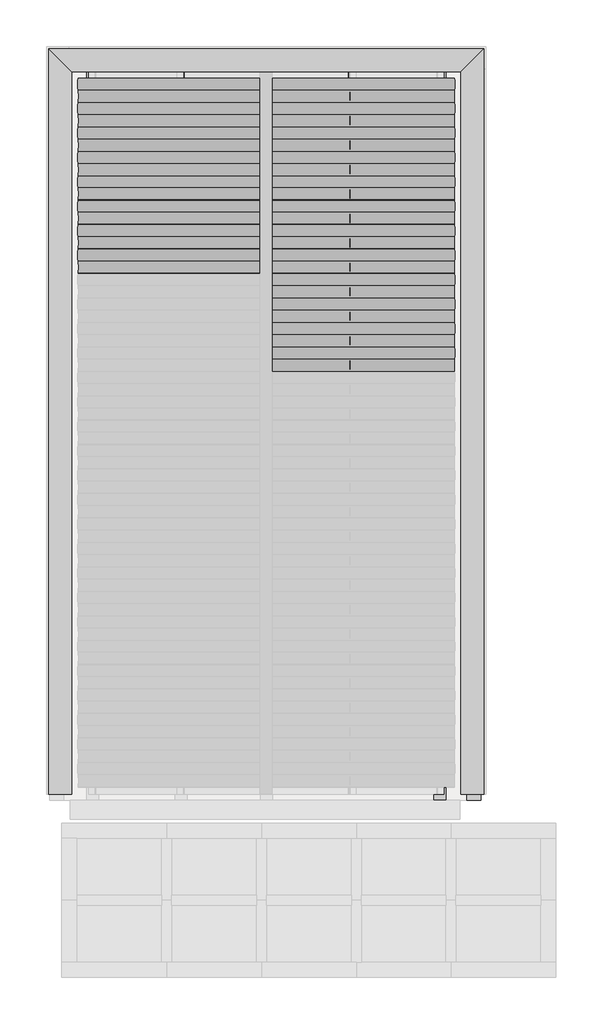
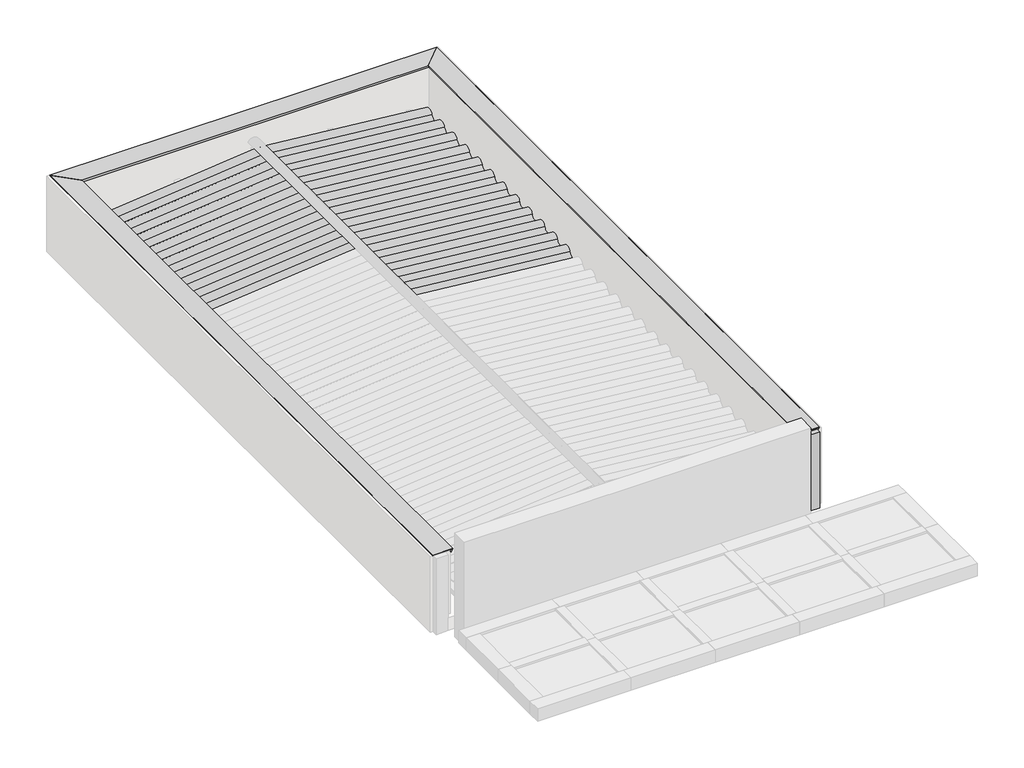
# One storey, part 3 of 3: 35 beams, 12 columns, 1 proxy.
"""IFC4 building model written with IfcOpenShell, lengths in millimetres."""

import ifcopenshell
import ifcopenshell.guid

model = None  # the IFC model being written
_history = None  # IfcOwnerHistory: only IFC2X3 demands one
_inside = {}  # id of a spatial element -> (the spatial element, [elements in it])
_under = {}  # id of a project, library or spatial element -> (it, [spatial elements below it])
_declared = {}  # id of a project -> (the project, [libraries it declares])
_typed = {}  # id of a type object -> (the type object, [elements of that type])
_made_of = {}  # id of a material, layer set ... -> (it, [elements and type objects made of it])


def new_model(schema):
    """Start an empty IFC model of exactly this schema.

    Asked for "IFC4X3", IfcOpenShell would pick the latest addendum, in which some entities
    have other attributes; the version numbers below select the first issue.
    IFC2X3 requires an IfcOwnerHistory on every rooted entity: one is made here for all.
    """
    global model, _history
    if schema == "IFC4X3":
        model = ifcopenshell.file(schema_version=(4, 3, 0, 0))
    else:
        model = ifcopenshell.file(schema=schema)
    _inside.clear()
    _under.clear()
    _declared.clear()
    _typed.clear()
    _made_of.clear()
    _history = None
    if model.schema == "IFC2X3":
        org = make("IfcOrganization", Name="unknown")
        user = make(
            "IfcPersonAndOrganization",
            ThePerson=make("IfcPerson", FamilyName="unknown"),
            TheOrganization=org,
        )
        app = make(
            "IfcApplication",
            ApplicationDeveloper=org,
            Version="unknown",
            ApplicationFullName="unknown",
            ApplicationIdentifier="unknown",
        )
        _history = make(
            "IfcOwnerHistory",
            OwningUser=user,
            OwningApplication=app,
            ChangeAction="ADDED",
            CreationDate=0,
        )
    return model


def make(cls, **values):
    """One entity of the class cls with the attributes given. An attribute that is None is left unset."""
    return model.create_entity(
        cls, **{name: value for name, value in values.items() if value is not None}
    )


def rooted(cls, **values):
    """An entity with a GlobalId (a new one), such as an element, a storey or a relation."""
    return make(cls, GlobalId=ifcopenshell.guid.new(), OwnerHistory=_history, **values)


def si_unit(unit_type, name, prefix=None):
    """IfcSIUnit, for example si_unit("LENGTHUNIT", "METRE", prefix="MILLI")."""
    return make("IfcSIUnit", UnitType=unit_type, Prefix=prefix, Name=name)


def assignment(units):
    """IfcUnitAssignment: the units of a project."""
    return None if units is None else make("IfcUnitAssignment", Units=units)


def point(xyz):
    """IfcCartesianPoint."""
    return None if xyz is None else make("IfcCartesianPoint", Coordinates=xyz)


def direction(xyz):
    """IfcDirection."""
    return None if xyz is None else make("IfcDirection", DirectionRatios=xyz)


def frame(location, z_axis=None, x_axis=None):
    """IfcAxis2Placement3D, a coordinate frame: its origin and axes. An axis left out is left unset."""
    return make(
        "IfcAxis2Placement3D",
        Location=point(location),
        Axis=direction(z_axis),
        RefDirection=direction(x_axis),
    )


def frame_2d(location, x_axis=None):
    """IfcAxis2Placement2D, a coordinate frame in the plane: its origin and x axis."""
    return make(
        "IfcAxis2Placement2D", Location=point(location), RefDirection=direction(x_axis)
    )


def origin():
    """The frame at (0, 0, 0) with its axes left unset."""
    return frame((0.0, 0.0, 0.0))


def place(relative_to, where):
    """IfcLocalPlacement: puts the frame where relative to a parent placement (None: the world)."""
    return make(
        "IfcLocalPlacement", PlacementRelTo=relative_to, RelativePlacement=where
    )


def context(
    kind, dimensions, precision=None, world=None, true_north=None, identifier=None
):
    """IfcGeometricRepresentationContext, for example the 3D "Model" context."""
    return make(
        "IfcGeometricRepresentationContext",
        ContextIdentifier=identifier,
        ContextType=kind,
        CoordinateSpaceDimension=dimensions,
        Precision=precision,
        WorldCoordinateSystem=world,
        TrueNorth=true_north,
    )


def project(units=None, contexts=None):
    """IfcProject with its units and contexts."""
    return rooted(
        "IfcProject",
        Name="project",
        RepresentationContexts=contexts,
        UnitsInContext=assignment(units),
    )


def spatial(cls, under=None, at=None, **own):
    """A site, building, storey or space (cls), placed at a placement, below another one or the project."""
    s = rooted(cls, ObjectPlacement=at, **own)
    if under is not None:
        _under.setdefault(under.id(), (under, []))[1].append(s)
    return s


def polyline(points):
    """IfcPolyline through the points."""
    return make("IfcPolyline", Points=[point(p) for p in points])


def circle_curve(where, radius):
    """IfcCircle in the frame where."""
    return make("IfcCircle", Position=where, Radius=radius)


def trimmed(basis, trim1, trim2, sense, master):
    """IfcTrimmedCurve: the piece of a basis curve between two trims."""
    return make(
        "IfcTrimmedCurve",
        BasisCurve=basis,
        Trim1=trim1,
        Trim2=trim2,
        SenseAgreement=sense,
        MasterRepresentation=master,
    )


def segment(curve, same_sense, transition):
    """IfcCompositeCurveSegment."""
    return make(
        "IfcCompositeCurveSegment",
        Transition=transition,
        SameSense=same_sense,
        ParentCurve=curve,
    )


def composite_curve(segments, self_intersect=None):
    """IfcCompositeCurve: segments joined end to end."""
    return make("IfcCompositeCurve", Segments=segments, SelfIntersect=self_intersect)


def outline(outer, holes=None, kind="AREA"):
    """IfcArbitraryClosedProfileDef: a profile drawn as a closed curve; with holes, ...WithVoids."""
    if holes is None:
        return make("IfcArbitraryClosedProfileDef", ProfileType=kind, OuterCurve=outer)
    return make(
        "IfcArbitraryProfileDefWithVoids",
        ProfileType=kind,
        OuterCurve=outer,
        InnerCurves=holes,
    )


def extrude(swept, where, along, depth):
    """IfcExtrudedAreaSolid: the profile swept, set in the frame where, extruded along a direction by depth."""
    return make(
        "IfcExtrudedAreaSolid",
        SweptArea=swept,
        Position=where,
        ExtrudedDirection=direction(along),
        Depth=depth,
    )


def faces_of(points, faces, orient=None, outer=None):
    """IfcFace entities. A face is a list of loops; a loop is a list of indices into points, from 0.

    orient and outer hold one flag for each loop. By default every Orientation is true, the
    first loop of a face is its IfcFaceOuterBound and the others are IfcFaceBound.
    """
    made = []
    for i, loops in enumerate(faces):
        bounds = []
        for j, loop in enumerate(loops):
            is_outer = j == 0 if outer is None else outer[i][j]
            bounds.append(
                make(
                    "IfcFaceOuterBound" if is_outer else "IfcFaceBound",
                    Bound=make("IfcPolyLoop", Polygon=[points[k] for k in loop]),
                    Orientation=True if orient is None else orient[i][j],
                )
            )
        made.append(make("IfcFace", Bounds=bounds))
    return made


def faceted_brep(points, faces, orient=None, outer=None, voids=None):
    """IfcFacetedBrep: a solid bounded by flat faces; with voids (closed shells), ...WithVoids."""
    shared = [point(p) for p in points]
    hull = make("IfcClosedShell", CfsFaces=faces_of(shared, faces, orient, outer))
    if voids is None:
        return make("IfcFacetedBrep", Outer=hull)
    return make(
        "IfcFacetedBrepWithVoids",
        Outer=hull,
        Voids=[
            make(cls, CfsFaces=faces_of(shared, fs, o, b)) for cls, fs, o, b in voids
        ],
    )


def shape(context_of_items, identifier, shape_type, items):
    """IfcShapeRepresentation: the items that make up one representation, for example the "Body"."""
    return make(
        "IfcShapeRepresentation",
        ContextOfItems=context_of_items,
        RepresentationIdentifier=identifier,
        RepresentationType=shape_type,
        Items=items,
    )


def source(mapping_origin, context_of_items, identifier, shape_type, items):
    """IfcRepresentationMap: a shape defined once, which mapped items show again and again."""
    return make(
        "IfcRepresentationMap",
        MappingOrigin=mapping_origin,
        MappedRepresentation=shape(context_of_items, identifier, shape_type, items),
    )


def transform(
    local_origin,
    x_axis=None,
    y_axis=None,
    z_axis=None,
    scale=None,
    scale2=None,
    scale3=None,
    uniform=True,
):
    """IfcCartesianTransformationOperator3D, or its non-uniform kind. x_axis, y_axis, z_axis: its Axis1, 2, 3."""
    if uniform:
        return make(
            "IfcCartesianTransformationOperator3D",
            Axis1=direction(x_axis),
            Axis2=direction(y_axis),
            LocalOrigin=point(local_origin),
            Scale=scale,
            Axis3=direction(z_axis),
        )
    return make(
        "IfcCartesianTransformationOperator3DnonUniform",
        Axis1=direction(x_axis),
        Axis2=direction(y_axis),
        LocalOrigin=point(local_origin),
        Scale=scale,
        Axis3=direction(z_axis),
        Scale2=scale2,
        Scale3=scale3,
    )


def mapped(mapping_source, mapping_target):
    """IfcMappedItem: shows the shape of a source again, moved by a transform."""
    return make(
        "IfcMappedItem", MappingSource=mapping_source, MappingTarget=mapping_target
    )


def made_of(thing, what):
    """Note that an element or type object is made of a material, layer set ...; save() writes the relation."""
    if what is not None:
        _made_of.setdefault(what.id(), (what, []))[1].append(thing)
    return thing


def element(
    cls,
    number,
    at=None,
    inside=None,
    cuts=None,
    type_object=None,
    material=None,
    context=None,
    identifier="Body",
    shape_type=None,
    held_by="IfcProductDefinitionShape",
    body=None,
    shapes=None,
    **own,
):
    """One element of the class cls, such as IfcWall. Its Tag is "e" and its number.

    at: its placement. inside: the storey or other place that contains it. cuts: it is an
    opening in that element (IfcRelVoidsElement). A single representation is given by context,
    identifier, shape_type and body (its items); several are given by shapes. held_by: the class
    of the entity that holds the representations. save() writes the other relations.
    """
    e = rooted(cls, Tag="e%d" % number, ObjectPlacement=at, **own)
    if body is not None:
        shapes = [shape(context, identifier, shape_type, body)]
    if shapes is not None:
        e.Representation = make(held_by, Representations=shapes)
    if inside is not None:
        _inside.setdefault(inside.id(), (inside, []))[1].append(e)
    if cuts is not None:
        rooted(
            "IfcRelVoidsElement", RelatingBuildingElement=cuts, RelatedOpeningElement=e
        )
    if type_object is not None:
        _typed.setdefault(type_object.id(), (type_object, []))[1].append(e)
    return made_of(e, material)


def aggregate(whole, parts):
    """IfcRelAggregates: a whole, such as a stair, and the parts it consists of."""
    return rooted("IfcRelAggregates", RelatingObject=whole, RelatedObjects=parts)


def save(model, path):
    """Write the relations noted so far, then the file.

    IfcRelAggregates (storeys below a building ...), IfcRelContainedInSpatialStructure (elements
    in a storey), IfcRelDefinesByType, IfcRelAssociatesMaterial and IfcRelDeclares: one each for
    every whole, place, type object, material and project.
    """
    for whole, parts in _under.values():
        aggregate(whole, parts)
    for where, things in _inside.values():
        rooted(
            "IfcRelContainedInSpatialStructure",
            RelatedElements=things,
            RelatingStructure=where,
        )
    for kind, things in _typed.values():
        rooted("IfcRelDefinesByType", RelatedObjects=things, RelatingType=kind)
    for what, things in _made_of.values():
        rooted("IfcRelAssociatesMaterial", RelatedObjects=things, RelatingMaterial=what)
    for by, libraries in _declared.values():
        rooted("IfcRelDeclares", RelatingContext=by, RelatedDefinitions=libraries)
    model.write(path)


def column_1cffec27(model_context):
    return source(origin(), model_context, "Body", "SweptSolid", [
        extrude(outline(polyline([(30.0, 80.0), (30.0, -80.0), (-30.0, -80.0), (-30.0, 80.0), (30.0, 80.0)])), frame((0.0, 0.0, 3110.0), z_axis=(0.0, 0.0, 1.0), x_axis=(1.0, 0.0, 0.0)), (0.0, 0.0, 1.0), 238.0),
    ])


def column_35730ad5(model_context):
    return source(origin(), model_context, "Body", "SweptSolid", [
        extrude(outline(polyline([(30.0, 80.0), (30.0, -80.0), (-30.0, -80.0), (-30.0, 80.0), (30.0, 80.0)])), frame((0.0, 0.0, 3110.0), z_axis=(0.0, 0.0, 1.0), x_axis=(1.0, 0.0, 0.0)), (0.0, 0.0, 1.0), 197.9),
    ])


def column_00c463e4(model_context):
    return source(origin(), model_context, "Body", "SweptSolid", [
        extrude(outline(polyline([(30.0, 80.0), (30.0, -80.0), (-30.0, -80.0), (-30.0, 80.0), (30.0, 80.0)])), frame((0.0, 0.0, 3110.0), z_axis=(0.0, 0.0, 1.0), x_axis=(1.0, 0.0, 0.0)), (0.0, 0.0, 1.0), 109.8),
    ])


model = new_model("IFC4")

# Units and contexts
model_context = context("Model", 3, world=origin())
ifc_project = project(units=[si_unit("LENGTHUNIT", "METRE", prefix="MILLI")], contexts=[model_context])

# Site, building, storey
site = spatial("IfcSite", under=ifc_project)
building = spatial("IfcBuilding", under=site)
storey = spatial("IfcBuildingStorey", under=building, Name="COB. GARAGEM", Elevation=3050.0)

# Beams
placement = place(None, origin())
element("IfcBeam", 1, ObjectType="Madeira de lei : Berço 6x12cm", at=placement, inside=storey, context=model_context, shape_type="SweptSolid", body=[
    extrude(outline(polyline([(-9620.281307, 6423.9300153), (-9500.281307, 6423.9300153), (-9500.281307, 4423.9300153), (-9620.281307, 4423.9300153), (-9620.281307, 6423.9300153)])), frame((0.0, 0.0, 3050.0), z_axis=(0.0, 0.0, 1.0), x_axis=(1.0, 0.0, 0.0)), (0.0, 0.0, 1.0), 60.0),
])
element("IfcBeam", 2, ObjectType="Madeira de lei : Berço 6x12cm", at=placement, inside=storey, context=model_context, shape_type="SweptSolid", body=[
    extrude(outline(polyline([(-9620.281307, 7083.9300153), (-9500.281307, 7083.9300153), (-9500.281307, 6423.9300153), (-9620.281307, 6423.9300153), (-9620.281307, 7083.9300153)])), frame((0.0, 0.0, 3050.0), z_axis=(0.0, 0.0, 1.0), x_axis=(1.0, 0.0, 0.0)), (0.0, 0.0, 1.0), 60.0),
])
element("IfcBeam", 3, ObjectType="Madeira de lei : Berço 6x12cm", at=placement, inside=storey, context=model_context, shape_type="SweptSolid", body=[
    extrude(outline(polyline([(-8767.0824227, 6423.9300153), (-8647.0824227, 6423.9300153), (-8647.0824227, 4423.9300153), (-8767.0824227, 4423.9300153), (-8767.0824227, 6423.9300153)])), frame((0.0, 0.0, 3050.0), z_axis=(0.0, 0.0, 1.0), x_axis=(1.0, 0.0, 0.0)), (0.0, 0.0, 1.0), 60.0),
])
element("IfcBeam", 4, ObjectType="Madeira de lei : Berço 6x12cm", at=placement, inside=storey, context=model_context, shape_type="SweptSolid", body=[
    extrude(outline(polyline([(-8767.0824227, 7083.9300153), (-8647.0824227, 7083.9300153), (-8647.0824227, 6423.9300153), (-8767.0824227, 6423.9300153), (-8767.0824227, 7083.9300153)])), frame((0.0, 0.0, 3050.0), z_axis=(0.0, 0.0, 1.0), x_axis=(1.0, 0.0, 0.0)), (0.0, 0.0, 1.0), 60.0),
])
element("IfcBeam", 5, ObjectType="Madeira de lei : Berço 6x12cm", at=placement, inside=storey, context=model_context, shape_type="SweptSolid", body=[
    extrude(outline(polyline([(-7884.0324227, 4423.9300153), (-7764.0324227, 4423.9300153), (-7764.0324227, 2423.9300153), (-7884.0324227, 2423.9300153), (-7884.0324227, 4423.9300153)])), frame((0.0, 0.0, 3050.0), z_axis=(0.0, 0.0, 1.0), x_axis=(1.0, 0.0, 0.0)), (0.0, 0.0, 1.0), 60.0),
])
element("IfcBeam", 6, ObjectType="Madeira de lei : Berço 6x12cm", at=placement, inside=storey, context=model_context, shape_type="SweptSolid", body=[
    extrude(outline(polyline([(-7884.0324227, 6423.9300153), (-7764.0324227, 6423.9300153), (-7764.0324227, 4423.9300153), (-7884.0324227, 4423.9300153), (-7884.0324227, 6423.9300153)])), frame((0.0, 0.0, 3050.0), z_axis=(0.0, 0.0, 1.0), x_axis=(1.0, 0.0, 0.0)), (0.0, 0.0, 1.0), 60.0),
])
element("IfcBeam", 7, ObjectType="Madeira de lei : Berço 6x12cm", at=placement, inside=storey, context=model_context, shape_type="SweptSolid", body=[
    extrude(outline(polyline([(-7884.0324227, 2423.9300153), (-7764.0324227, 2423.9300153), (-7764.0324227, 423.9300153), (-7884.0324227, 423.9300153), (-7884.0324227, 2423.9300153)])), frame((0.0, 0.0, 3050.0), z_axis=(0.0, 0.0, 1.0), x_axis=(1.0, 0.0, 0.0)), (0.0, 0.0, 1.0), 60.0),
])
element("IfcBeam", 8, ObjectType="Madeira de lei : Berço 6x12cm", at=placement, inside=storey, context=model_context, shape_type="SweptSolid", body=[
    extrude(outline(polyline([(-7884.0324227, 7083.9300153), (-7764.0324227, 7083.9300153), (-7764.0324227, 6423.9300153), (-7884.0324227, 6423.9300153), (-7884.0324227, 7083.9300153)])), frame((0.0, 0.0, 3050.0), z_axis=(0.0, 0.0, 1.0), x_axis=(1.0, 0.0, 0.0)), (0.0, 0.0, 1.0), 60.0),
])
element("IfcBeam", 9, ObjectType="Madeira de lei : Berço 6x12cm", at=placement, inside=storey, context=model_context, shape_type="SweptSolid", body=[
    extrude(outline(polyline([(-7884.0324227, 423.9300153), (-7764.0324227, 423.9300153), (-7764.0324227, -236.0699847), (-7884.0324227, -236.0699847), (-7884.0324227, 423.9300153)])), frame((0.0, 0.0, 3050.0), z_axis=(0.0, 0.0, 1.0), x_axis=(1.0, 0.0, 0.0)), (0.0, 0.0, 1.0), 60.0),
])
element("IfcBeam", 10, ObjectType="Madeira de lei : Berço 6x12cm", at=placement, inside=storey, context=model_context, shape_type="SweptSolid", body=[
    extrude(outline(polyline([(-10473.4801913, 6423.9300153), (-10353.4801913, 6423.9300153), (-10353.4801913, 4423.9300153), (-10473.4801913, 4423.9300153), (-10473.4801913, 6423.9300153)])), frame((0.0, 0.0, 3050.0), z_axis=(0.0, 0.0, 1.0), x_axis=(1.0, 0.0, 0.0)), (0.0, 0.0, 1.0), 60.0),
])
element("IfcBeam", 11, ObjectType="Madeira de lei : Berço 6x12cm", at=placement, inside=storey, context=model_context, shape_type="SweptSolid", body=[
    extrude(outline(polyline([(-10473.4801913, 7083.9300153), (-10353.4801913, 7083.9300153), (-10353.4801913, 6423.9300153), (-10473.4801913, 6423.9300153), (-10473.4801913, 7083.9300153)])), frame((0.0, 0.0, 3050.0), z_axis=(0.0, 0.0, 1.0), x_axis=(1.0, 0.0, 0.0)), (0.0, 0.0, 1.0), 60.0),
])
element("IfcBeam", 12, ObjectType="Madeira de lei : Berço 6x12cm", at=placement, inside=storey, context=model_context, shape_type="SweptSolid", body=[
    extrude(outline(polyline([(-11356.5301913, 6423.9300153), (-11236.5301913, 6423.9300153), (-11236.5301913, 4423.9300153), (-11356.5301913, 4423.9300153), (-11356.5301913, 6423.9300153)])), frame((0.0, 0.0, 3050.0), z_axis=(0.0, 0.0, 1.0), x_axis=(1.0, 0.0, 0.0)), (0.0, 0.0, 1.0), 60.0),
])
element("IfcBeam", 13, ObjectType="Madeira de lei : Berço 6x12cm", at=placement, inside=storey, context=model_context, shape_type="SweptSolid", body=[
    extrude(outline(polyline([(-11356.5301913, 7083.9300153), (-11236.5301913, 7083.9300153), (-11236.5301913, 6423.9300153), (-11356.5301913, 6423.9300153), (-11356.5301913, 7083.9300153)])), frame((0.0, 0.0, 3050.0), z_axis=(0.0, 0.0, 1.0), x_axis=(1.0, 0.0, 0.0)), (0.0, 0.0, 1.0), 60.0),
])
element("IfcBeam", 14, ObjectType="TQS - Viga retangular : 14.0 x 90.0", at=placement, inside=storey, context=model_context, shape_type="Brep", body=[
    faceted_brep([(-7712.281307, 7134.4300153, 3800.0), (-7712.281307, 7274.4300153, 3800.0), (-11430.281307, 7274.4300153, 3800.0), (-11430.281307, 7134.4300153, 3800.0), (-7712.281307, 7134.4300153, 2900.0), (-7712.281307, 7134.4300153, 3050.0), (-11430.281307, 7134.4300153, 3050.0), (-11430.281307, 7134.4300153, 2900.0), (-7712.281307, 7274.4300153, 2900.0), (-11430.281307, 7274.4300153, 2900.0)], [[[0, 1, 2, 3]], [[4, 5, 0, 3, 6, 7]], [[8, 4, 7, 9]], [[1, 8, 9, 2]], [[2, 9, 7, 6, 3]], [[1, 0, 5, 4, 8]]]),
])
element("IfcBeam", 15, ObjectType="TQS - Viga retangular : 14.0 x 90.0", at=placement, inside=storey, context=model_context, shape_type="Brep", body=[
    faceted_brep([(-7412.281307, 7084.4300153, 3800.0), (-7552.281307, 7084.4300153, 3800.0), (-7552.281307, -234.5699847, 3800.0), (-7412.281307, -234.5699847, 3800.0), (-7412.281307, 7084.4300153, 2900.0), (-7412.281307, -234.5699847, 2900.0), (-7552.281307, 7084.4300153, 2900.0), (-7552.281307, -234.5699847, 2900.0), (-7552.281307, 7084.4300153, 3050.0), (-7552.281307, -234.5699847, 3050.0)], [[[0, 1, 2, 3]], [[4, 0, 3, 5]], [[6, 4, 5, 7]], [[1, 8, 6, 7, 9, 2]], [[2, 9, 7, 5, 3]], [[1, 0, 4, 6, 8]]]),
])
element("IfcBeam", 16, ObjectType="Telha Ondulada : Fibrocimento", at=placement, inside=storey, context=model_context, shape_type="SweptSolid", body=[
    extrude(outline(composite_curve([segment(trimmed(circle_curve(frame_2d((-58.7002979, -53.2060538)), 66.7939461), [point((-29.350149, 6.7939462))], [point((-29.350149, -113.2060538))], False, "CARTESIAN"), True, "CONTINUOUS"), segment(polyline([(-29.350149, -113.2060538), (-31.5472155, -108.7146288)]), True, "CONTINUOUS"), segment(trimmed(circle_curve(frame_2d((-58.7002979, -53.2060538)), 61.7939461), [point((-31.5472155, -108.7146288))], [point((-31.5472155, 2.3025211))], True, "CARTESIAN"), True, "CONTINUOUS"), segment(trimmed(circle_curve(frame_2d((0.0, 66.7939462)), 71.7939461), [point((-31.5472155, 2.3025211))], [point((-31.5472155, 131.2853712))], False, "CARTESIAN"), True, "CONTINUOUS"), segment(polyline([(-31.5472155, 131.2853712), (-29.350149, 126.7939462)]), True, "CONTINUOUS"), segment(trimmed(circle_curve(frame_2d((0.0, 66.7939462)), 66.7939461), [point((-29.350149, 126.7939462))], [point((-29.350149, 6.7939462))], True, "CARTESIAN"), True, "CONTINUOUS")], self_intersect=False)), frame((-11446.918865, 5163.326948, 3394.3067746), z_axis=(0.9950371902099892, 0.0, 0.09950371902099937), x_axis=(-0.09950371902099937, 0.0, 0.9950371902099892)), (0.0, 0.0, 1.0), 1886.8678854),
])
element("IfcBeam", 17, ObjectType="Telha Ondulada : Fibrocimento", at=placement, inside=storey, context=model_context, shape_type="SweptSolid", body=[
    extrude(outline(composite_curve([segment(trimmed(circle_curve(frame_2d((-58.7002979, -53.2060538)), 66.7939461), [point((-29.350149, 6.7939462))], [point((-29.350149, -113.2060538))], False, "CARTESIAN"), True, "CONTINUOUS"), segment(polyline([(-29.350149, -113.2060538), (-31.5472155, -108.7146288)]), True, "CONTINUOUS"), segment(trimmed(circle_curve(frame_2d((-58.7002979, -53.2060538)), 61.7939461), [point((-31.5472155, -108.7146288))], [point((-31.5472155, 2.3025211))], True, "CARTESIAN"), True, "CONTINUOUS"), segment(trimmed(circle_curve(frame_2d((0.0, 66.7939462)), 71.7939461), [point((-31.5472155, 2.3025211))], [point((-31.5472155, 131.2853712))], False, "CARTESIAN"), True, "CONTINUOUS"), segment(polyline([(-31.5472155, 131.2853712), (-29.350149, 126.7939462)]), True, "CONTINUOUS"), segment(trimmed(circle_curve(frame_2d((0.0, 66.7939462)), 66.7939461), [point((-29.350149, 126.7939462))], [point((-29.350149, 6.7939462))], True, "CARTESIAN"), True, "CONTINUOUS")], self_intersect=False)), frame((-11446.918865, 5407.826948, 3394.3067746), z_axis=(0.9950371902099892, 0.0, 0.09950371902099972), x_axis=(-0.09950371902099972, 0.0, 0.9950371902099892)), (0.0, 0.0, 1.0), 1886.8678854),
])
element("IfcBeam", 18, ObjectType="Telha Ondulada : Fibrocimento", at=placement, inside=storey, context=model_context, shape_type="SweptSolid", body=[
    extrude(outline(composite_curve([segment(trimmed(circle_curve(frame_2d((-58.7002979, -53.2060538)), 66.7939461), [point((-29.350149, 6.7939462))], [point((-29.350149, -113.2060538))], False, "CARTESIAN"), True, "CONTINUOUS"), segment(polyline([(-29.350149, -113.2060538), (-31.5472155, -108.7146288)]), True, "CONTINUOUS"), segment(trimmed(circle_curve(frame_2d((-58.7002979, -53.2060538)), 61.7939461), [point((-31.5472155, -108.7146288))], [point((-31.5472155, 2.3025211))], True, "CARTESIAN"), True, "CONTINUOUS"), segment(trimmed(circle_curve(frame_2d((0.0, 66.7939462)), 71.7939461), [point((-31.5472155, 2.3025211))], [point((-31.5472155, 131.2853712))], False, "CARTESIAN"), True, "CONTINUOUS"), segment(polyline([(-31.5472155, 131.2853712), (-29.350149, 126.7939462)]), True, "CONTINUOUS"), segment(trimmed(circle_curve(frame_2d((0.0, 66.7939462)), 66.7939461), [point((-29.350149, 126.7939462))], [point((-29.350149, 6.7939462))], True, "CARTESIAN"), True, "CONTINUOUS")], self_intersect=False)), frame((-11446.918865, 5652.326948, 3394.3067746), z_axis=(0.9950371902099892, 0.0, 0.09950371902099954), x_axis=(-0.09950371902099954, 0.0, 0.9950371902099892)), (0.0, 0.0, 1.0), 1886.8678854),
])
element("IfcBeam", 19, ObjectType="Telha Ondulada : Fibrocimento", at=placement, inside=storey, context=model_context, shape_type="SweptSolid", body=[
    extrude(outline(composite_curve([segment(trimmed(circle_curve(frame_2d((-58.7002979, -53.2060538)), 66.7939461), [point((-29.350149, 6.7939462))], [point((-29.350149, -113.2060538))], False, "CARTESIAN"), True, "CONTINUOUS"), segment(polyline([(-29.350149, -113.2060538), (-31.5472155, -108.7146288)]), True, "CONTINUOUS"), segment(trimmed(circle_curve(frame_2d((-58.7002979, -53.2060538)), 61.7939461), [point((-31.5472155, -108.7146288))], [point((-31.5472155, 2.3025211))], True, "CARTESIAN"), True, "CONTINUOUS"), segment(trimmed(circle_curve(frame_2d((0.0, 66.7939462)), 71.7939461), [point((-31.5472155, 2.3025211))], [point((-31.5472155, 131.2853712))], False, "CARTESIAN"), True, "CONTINUOUS"), segment(polyline([(-31.5472155, 131.2853712), (-29.350149, 126.7939462)]), True, "CONTINUOUS"), segment(trimmed(circle_curve(frame_2d((0.0, 66.7939462)), 66.7939461), [point((-29.350149, 126.7939462))], [point((-29.350149, 6.7939462))], True, "CARTESIAN"), True, "CONTINUOUS")], self_intersect=False)), frame((-11446.918865, 5896.826948, 3394.3067746), z_axis=(0.9950371902099892, 0.0, 0.09950371902099932), x_axis=(-0.09950371902099932, 0.0, 0.9950371902099892)), (0.0, 0.0, 1.0), 1886.8678854),
])
element("IfcBeam", 20, ObjectType="Telha Ondulada : Fibrocimento", at=placement, inside=storey, context=model_context, shape_type="SweptSolid", body=[
    extrude(outline(composite_curve([segment(trimmed(circle_curve(frame_2d((-58.7002979, -53.2060538)), 66.7939461), [point((-29.350149, 6.7939462))], [point((-29.350149, -113.2060538))], False, "CARTESIAN"), True, "CONTINUOUS"), segment(polyline([(-29.350149, -113.2060538), (-31.5472155, -108.7146288)]), True, "CONTINUOUS"), segment(trimmed(circle_curve(frame_2d((-58.7002979, -53.2060538)), 61.7939461), [point((-31.5472155, -108.7146288))], [point((-31.5472155, 2.3025211))], True, "CARTESIAN"), True, "CONTINUOUS"), segment(trimmed(circle_curve(frame_2d((0.0, 66.7939462)), 71.7939461), [point((-31.5472155, 2.3025211))], [point((-31.5472155, 131.2853712))], False, "CARTESIAN"), True, "CONTINUOUS"), segment(polyline([(-31.5472155, 131.2853712), (-29.350149, 126.7939462)]), True, "CONTINUOUS"), segment(trimmed(circle_curve(frame_2d((0.0, 66.7939462)), 66.7939461), [point((-29.350149, 126.7939462))], [point((-29.350149, 6.7939462))], True, "CARTESIAN"), True, "CONTINUOUS")], self_intersect=False)), frame((-11446.918865, 6141.326948, 3394.3067746), z_axis=(0.9950371902099892, 0.0, 0.09950371902099943), x_axis=(-0.09950371902099943, 0.0, 0.9950371902099892)), (0.0, 0.0, 1.0), 1886.8678854),
])
element("IfcBeam", 21, ObjectType="Telha Ondulada : Fibrocimento", at=placement, inside=storey, context=model_context, shape_type="SweptSolid", body=[
    extrude(outline(composite_curve([segment(trimmed(circle_curve(frame_2d((-58.7002979, -53.2060538)), 66.7939461), [point((-29.350149, 6.7939462))], [point((-29.350149, -113.2060538))], False, "CARTESIAN"), True, "CONTINUOUS"), segment(polyline([(-29.350149, -113.2060538), (-31.5472155, -108.7146288)]), True, "CONTINUOUS"), segment(trimmed(circle_curve(frame_2d((-58.7002979, -53.2060538)), 61.7939461), [point((-31.5472155, -108.7146288))], [point((-31.5472155, 2.3025211))], True, "CARTESIAN"), True, "CONTINUOUS"), segment(trimmed(circle_curve(frame_2d((0.0, 66.7939462)), 71.7939461), [point((-31.5472155, 2.3025211))], [point((-31.5472155, 131.2853712))], False, "CARTESIAN"), True, "CONTINUOUS"), segment(polyline([(-31.5472155, 131.2853712), (-29.350149, 126.7939462)]), True, "CONTINUOUS"), segment(trimmed(circle_curve(frame_2d((0.0, 66.7939462)), 66.7939461), [point((-29.350149, 126.7939462))], [point((-29.350149, 6.7939462))], True, "CARTESIAN"), True, "CONTINUOUS")], self_intersect=False)), frame((-11446.918865, 6385.826948, 3394.3067746), z_axis=(0.9950371902099892, 0.0, 0.09950371902099919), x_axis=(-0.09950371902099919, 0.0, 0.9950371902099892)), (0.0, 0.0, 1.0), 1886.8678854),
])
element("IfcBeam", 22, ObjectType="Telha Ondulada : Fibrocimento", at=placement, inside=storey, context=model_context, shape_type="SweptSolid", body=[
    extrude(outline(composite_curve([segment(trimmed(circle_curve(frame_2d((-58.7002979, -53.2060538)), 66.7939461), [point((-29.350149, 6.7939462))], [point((-29.350149, -113.2060538))], False, "CARTESIAN"), True, "CONTINUOUS"), segment(polyline([(-29.350149, -113.2060538), (-31.5472155, -108.7146288)]), True, "CONTINUOUS"), segment(trimmed(circle_curve(frame_2d((-58.7002979, -53.2060538)), 61.7939461), [point((-31.5472155, -108.7146288))], [point((-31.5472155, 2.3025211))], True, "CARTESIAN"), True, "CONTINUOUS"), segment(trimmed(circle_curve(frame_2d((0.0, 66.7939462)), 71.7939461), [point((-31.5472155, 2.3025211))], [point((-31.5472155, 131.2853712))], False, "CARTESIAN"), True, "CONTINUOUS"), segment(polyline([(-31.5472155, 131.2853712), (-29.350149, 126.7939462)]), True, "CONTINUOUS"), segment(trimmed(circle_curve(frame_2d((0.0, 66.7939462)), 66.7939461), [point((-29.350149, 126.7939462))], [point((-29.350149, 6.7939462))], True, "CARTESIAN"), True, "CONTINUOUS")], self_intersect=False)), frame((-11446.918865, 6630.326948, 3394.3067746), z_axis=(0.9950371902099892, 0.0, 0.09950371902099925), x_axis=(-0.09950371902099925, 0.0, 0.9950371902099892)), (0.0, 0.0, 1.0), 1886.8678854),
])
element("IfcBeam", 23, ObjectType="Telha Ondulada : Fibrocimento", at=placement, inside=storey, context=model_context, shape_type="SweptSolid", body=[
    extrude(outline(composite_curve([segment(trimmed(circle_curve(frame_2d((-58.7002979, -53.2060538)), 66.7939461), [point((-29.350149, 6.7939462))], [point((-29.350149, -113.2060538))], False, "CARTESIAN"), True, "CONTINUOUS"), segment(polyline([(-29.350149, -113.2060538), (-31.5472155, -108.7146288)]), True, "CONTINUOUS"), segment(trimmed(circle_curve(frame_2d((-58.7002979, -53.2060538)), 61.7939461), [point((-31.5472155, -108.7146288))], [point((-31.5472155, 2.3025211))], True, "CARTESIAN"), True, "CONTINUOUS"), segment(trimmed(circle_curve(frame_2d((0.0, 66.7939462)), 71.7939461), [point((-31.5472155, 2.3025211))], [point((-31.5472155, 131.2853712))], False, "CARTESIAN"), True, "CONTINUOUS"), segment(polyline([(-31.5472155, 131.2853712), (-29.350149, 126.7939462)]), True, "CONTINUOUS"), segment(trimmed(circle_curve(frame_2d((0.0, 66.7939462)), 66.7939461), [point((-29.350149, 126.7939462))], [point((-29.350149, 6.7939462))], True, "CARTESIAN"), True, "CONTINUOUS")], self_intersect=False)), frame((-11446.918865, 6874.826948, 3394.3067746), z_axis=(0.9950371902099892, 0.0, 0.09950371902099937), x_axis=(-0.09950371902099937, 0.0, 0.9950371902099892)), (0.0, 0.0, 1.0), 1886.8678854),
])
element("IfcBeam", 24, ObjectType="Telha Ondulada : Fibrocimento", at=placement, inside=storey, context=model_context, shape_type="SweptSolid", body=[
    extrude(outline(composite_curve([segment(trimmed(circle_curve(frame_2d((0.0, 66.7939462)), 66.7939461), [point((29.350149, 6.7939462))], [point((29.350149, 126.7939462))], True, "CARTESIAN"), True, "CONTINUOUS"), segment(polyline([(29.350149, 126.7939462), (31.5472155, 131.2853712)]), True, "CONTINUOUS"), segment(trimmed(circle_curve(frame_2d((0.0, 66.7939462)), 71.7939461), [point((31.5472155, 131.2853712))], [point((31.5472155, 2.3025211))], False, "CARTESIAN"), True, "CONTINUOUS"), segment(trimmed(circle_curve(frame_2d((58.7002979, -53.2060538)), 61.7939461), [point((31.5472155, 2.3025211))], [point((31.5472155, -108.7146288))], True, "CARTESIAN"), True, "CONTINUOUS"), segment(polyline([(31.5472155, -108.7146288), (29.350149, -113.2060538)]), True, "CONTINUOUS"), segment(trimmed(circle_curve(frame_2d((58.7002979, -53.2060538)), 66.7939461), [point((29.350149, -113.2060538))], [point((29.350149, 6.7939462))], False, "CARTESIAN"), True, "CONTINUOUS")], self_intersect=False)), frame((-7673.6437489, 4185.326948, 3394.3067746), z_axis=(-0.9950371902099892, 0.0, 0.09950371902099965), x_axis=(-0.09950371902099965, 0.0, -0.9950371902099892)), (0.0, 0.0, 1.0), 1886.8678854),
])
element("IfcBeam", 25, ObjectType="Telha Ondulada : Fibrocimento", at=placement, inside=storey, context=model_context, shape_type="SweptSolid", body=[
    extrude(outline(composite_curve([segment(trimmed(circle_curve(frame_2d((0.0, 66.7939462)), 66.7939461), [point((29.350149, 6.7939462))], [point((29.350149, 126.7939462))], True, "CARTESIAN"), True, "CONTINUOUS"), segment(polyline([(29.350149, 126.7939462), (31.5472155, 131.2853712)]), True, "CONTINUOUS"), segment(trimmed(circle_curve(frame_2d((0.0, 66.7939462)), 71.7939461), [point((31.5472155, 131.2853712))], [point((31.5472155, 2.3025211))], False, "CARTESIAN"), True, "CONTINUOUS"), segment(trimmed(circle_curve(frame_2d((58.7002979, -53.2060538)), 61.7939461), [point((31.5472155, 2.3025211))], [point((31.5472155, -108.7146288))], True, "CARTESIAN"), True, "CONTINUOUS"), segment(polyline([(31.5472155, -108.7146288), (29.350149, -113.2060538)]), True, "CONTINUOUS"), segment(trimmed(circle_curve(frame_2d((58.7002979, -53.2060538)), 66.7939461), [point((29.350149, -113.2060538))], [point((29.350149, 6.7939462))], False, "CARTESIAN"), True, "CONTINUOUS")], self_intersect=False)), frame((-7673.6437489, 4429.826948, 3394.3067746), z_axis=(-0.9950371902099892, 0.0, 0.09950371902099965), x_axis=(-0.09950371902099965, 0.0, -0.9950371902099892)), (0.0, 0.0, 1.0), 1886.8678854),
])
element("IfcBeam", 26, ObjectType="Telha Ondulada : Fibrocimento", at=placement, inside=storey, context=model_context, shape_type="SweptSolid", body=[
    extrude(outline(composite_curve([segment(trimmed(circle_curve(frame_2d((0.0, 66.7939462)), 66.7939461), [point((29.350149, 6.7939462))], [point((29.350149, 126.7939462))], True, "CARTESIAN"), True, "CONTINUOUS"), segment(polyline([(29.350149, 126.7939462), (31.5472155, 131.2853712)]), True, "CONTINUOUS"), segment(trimmed(circle_curve(frame_2d((0.0, 66.7939462)), 71.7939461), [point((31.5472155, 131.2853712))], [point((31.5472155, 2.3025211))], False, "CARTESIAN"), True, "CONTINUOUS"), segment(trimmed(circle_curve(frame_2d((58.7002979, -53.2060538)), 61.7939461), [point((31.5472155, 2.3025211))], [point((31.5472155, -108.7146288))], True, "CARTESIAN"), True, "CONTINUOUS"), segment(polyline([(31.5472155, -108.7146288), (29.350149, -113.2060538)]), True, "CONTINUOUS"), segment(trimmed(circle_curve(frame_2d((58.7002979, -53.2060538)), 66.7939461), [point((29.350149, -113.2060538))], [point((29.350149, 6.7939462))], False, "CARTESIAN"), True, "CONTINUOUS")], self_intersect=False)), frame((-7673.6437489, 4674.326948, 3394.3067746), z_axis=(-0.9950371902099892, 0.0, 0.09950371902099965), x_axis=(-0.09950371902099965, 0.0, -0.9950371902099892)), (0.0, 0.0, 1.0), 1886.8678854),
])
element("IfcBeam", 27, ObjectType="Telha Ondulada : Fibrocimento", at=placement, inside=storey, context=model_context, shape_type="SweptSolid", body=[
    extrude(outline(composite_curve([segment(trimmed(circle_curve(frame_2d((0.0, 66.7939462)), 66.7939461), [point((29.350149, 6.7939462))], [point((29.350149, 126.7939462))], True, "CARTESIAN"), True, "CONTINUOUS"), segment(polyline([(29.350149, 126.7939462), (31.5472155, 131.2853712)]), True, "CONTINUOUS"), segment(trimmed(circle_curve(frame_2d((0.0, 66.7939462)), 71.7939461), [point((31.5472155, 131.2853712))], [point((31.5472155, 2.3025211))], False, "CARTESIAN"), True, "CONTINUOUS"), segment(trimmed(circle_curve(frame_2d((58.7002979, -53.2060538)), 61.7939461), [point((31.5472155, 2.3025211))], [point((31.5472155, -108.7146288))], True, "CARTESIAN"), True, "CONTINUOUS"), segment(polyline([(31.5472155, -108.7146288), (29.350149, -113.2060538)]), True, "CONTINUOUS"), segment(trimmed(circle_curve(frame_2d((58.7002979, -53.2060538)), 66.7939461), [point((29.350149, -113.2060538))], [point((29.350149, 6.7939462))], False, "CARTESIAN"), True, "CONTINUOUS")], self_intersect=False)), frame((-7673.6437489, 4918.826948, 3394.3067746), z_axis=(-0.9950371902099892, 0.0, 0.09950371902099965), x_axis=(-0.09950371902099965, 0.0, -0.9950371902099892)), (0.0, 0.0, 1.0), 1886.8678854),
])
element("IfcBeam", 28, ObjectType="Telha Ondulada : Fibrocimento", at=placement, inside=storey, context=model_context, shape_type="SweptSolid", body=[
    extrude(outline(composite_curve([segment(trimmed(circle_curve(frame_2d((0.0, 66.7939462)), 66.7939461), [point((29.350149, 6.7939462))], [point((29.350149, 126.7939462))], True, "CARTESIAN"), True, "CONTINUOUS"), segment(polyline([(29.350149, 126.7939462), (31.5472155, 131.2853712)]), True, "CONTINUOUS"), segment(trimmed(circle_curve(frame_2d((0.0, 66.7939462)), 71.7939461), [point((31.5472155, 131.2853712))], [point((31.5472155, 2.3025211))], False, "CARTESIAN"), True, "CONTINUOUS"), segment(trimmed(circle_curve(frame_2d((58.7002979, -53.2060538)), 61.7939461), [point((31.5472155, 2.3025211))], [point((31.5472155, -108.7146288))], True, "CARTESIAN"), True, "CONTINUOUS"), segment(polyline([(31.5472155, -108.7146288), (29.350149, -113.2060538)]), True, "CONTINUOUS"), segment(trimmed(circle_curve(frame_2d((58.7002979, -53.2060538)), 66.7939461), [point((29.350149, -113.2060538))], [point((29.350149, 6.7939462))], False, "CARTESIAN"), True, "CONTINUOUS")], self_intersect=False)), frame((-7673.6437489, 5163.326948, 3394.3067746), z_axis=(-0.9950371902099892, 0.0, 0.09950371902099965), x_axis=(-0.09950371902099965, 0.0, -0.9950371902099892)), (0.0, 0.0, 1.0), 1886.8678854),
])
element("IfcBeam", 29, ObjectType="Telha Ondulada : Fibrocimento", at=placement, inside=storey, context=model_context, shape_type="SweptSolid", body=[
    extrude(outline(composite_curve([segment(trimmed(circle_curve(frame_2d((0.0, 66.7939462)), 66.7939461), [point((29.350149, 6.7939462))], [point((29.350149, 126.7939462))], True, "CARTESIAN"), True, "CONTINUOUS"), segment(polyline([(29.350149, 126.7939462), (31.5472155, 131.2853712)]), True, "CONTINUOUS"), segment(trimmed(circle_curve(frame_2d((0.0, 66.7939462)), 71.7939461), [point((31.5472155, 131.2853712))], [point((31.5472155, 2.3025211))], False, "CARTESIAN"), True, "CONTINUOUS"), segment(trimmed(circle_curve(frame_2d((58.7002979, -53.2060538)), 61.7939461), [point((31.5472155, 2.3025211))], [point((31.5472155, -108.7146288))], True, "CARTESIAN"), True, "CONTINUOUS"), segment(polyline([(31.5472155, -108.7146288), (29.350149, -113.2060538)]), True, "CONTINUOUS"), segment(trimmed(circle_curve(frame_2d((58.7002979, -53.2060538)), 66.7939461), [point((29.350149, -113.2060538))], [point((29.350149, 6.7939462))], False, "CARTESIAN"), True, "CONTINUOUS")], self_intersect=False)), frame((-7673.6437489, 5407.826948, 3394.3067746), z_axis=(-0.9950371902099892, 0.0, 0.09950371902099965), x_axis=(-0.09950371902099965, 0.0, -0.9950371902099892)), (0.0, 0.0, 1.0), 1886.8678854),
])
element("IfcBeam", 30, ObjectType="Telha Ondulada : Fibrocimento", at=placement, inside=storey, context=model_context, shape_type="SweptSolid", body=[
    extrude(outline(composite_curve([segment(trimmed(circle_curve(frame_2d((0.0, 66.7939462)), 66.7939461), [point((29.350149, 6.7939462))], [point((29.350149, 126.7939462))], True, "CARTESIAN"), True, "CONTINUOUS"), segment(polyline([(29.350149, 126.7939462), (31.5472155, 131.2853712)]), True, "CONTINUOUS"), segment(trimmed(circle_curve(frame_2d((0.0, 66.7939462)), 71.7939461), [point((31.5472155, 131.2853712))], [point((31.5472155, 2.3025211))], False, "CARTESIAN"), True, "CONTINUOUS"), segment(trimmed(circle_curve(frame_2d((58.7002979, -53.2060538)), 61.7939461), [point((31.5472155, 2.3025211))], [point((31.5472155, -108.7146288))], True, "CARTESIAN"), True, "CONTINUOUS"), segment(polyline([(31.5472155, -108.7146288), (29.350149, -113.2060538)]), True, "CONTINUOUS"), segment(trimmed(circle_curve(frame_2d((58.7002979, -53.2060538)), 66.7939461), [point((29.350149, -113.2060538))], [point((29.350149, 6.7939462))], False, "CARTESIAN"), True, "CONTINUOUS")], self_intersect=False)), frame((-7673.6437489, 5652.326948, 3394.3067746), z_axis=(-0.9950371902099892, 0.0, 0.09950371902099965), x_axis=(-0.09950371902099965, 0.0, -0.9950371902099892)), (0.0, 0.0, 1.0), 1886.8678854),
])
element("IfcBeam", 31, ObjectType="Telha Ondulada : Fibrocimento", at=placement, inside=storey, context=model_context, shape_type="SweptSolid", body=[
    extrude(outline(composite_curve([segment(trimmed(circle_curve(frame_2d((0.0, 66.7939462)), 66.7939461), [point((29.350149, 6.7939462))], [point((29.350149, 126.7939462))], True, "CARTESIAN"), True, "CONTINUOUS"), segment(polyline([(29.350149, 126.7939462), (31.5472155, 131.2853712)]), True, "CONTINUOUS"), segment(trimmed(circle_curve(frame_2d((0.0, 66.7939462)), 71.7939461), [point((31.5472155, 131.2853712))], [point((31.5472155, 2.3025211))], False, "CARTESIAN"), True, "CONTINUOUS"), segment(trimmed(circle_curve(frame_2d((58.7002979, -53.2060538)), 61.7939461), [point((31.5472155, 2.3025211))], [point((31.5472155, -108.7146288))], True, "CARTESIAN"), True, "CONTINUOUS"), segment(polyline([(31.5472155, -108.7146288), (29.350149, -113.2060538)]), True, "CONTINUOUS"), segment(trimmed(circle_curve(frame_2d((58.7002979, -53.2060538)), 66.7939461), [point((29.350149, -113.2060538))], [point((29.350149, 6.7939462))], False, "CARTESIAN"), True, "CONTINUOUS")], self_intersect=False)), frame((-7673.6437489, 5896.826948, 3394.3067746), z_axis=(-0.9950371902099892, 0.0, 0.09950371902099965), x_axis=(-0.09950371902099965, 0.0, -0.9950371902099892)), (0.0, 0.0, 1.0), 1886.8678854),
])
element("IfcBeam", 32, ObjectType="Telha Ondulada : Fibrocimento", at=placement, inside=storey, context=model_context, shape_type="SweptSolid", body=[
    extrude(outline(composite_curve([segment(trimmed(circle_curve(frame_2d((0.0, 66.7939462)), 66.7939461), [point((29.350149, 6.7939462))], [point((29.350149, 126.7939462))], True, "CARTESIAN"), True, "CONTINUOUS"), segment(polyline([(29.350149, 126.7939462), (31.5472155, 131.2853712)]), True, "CONTINUOUS"), segment(trimmed(circle_curve(frame_2d((0.0, 66.7939462)), 71.7939461), [point((31.5472155, 131.2853712))], [point((31.5472155, 2.3025211))], False, "CARTESIAN"), True, "CONTINUOUS"), segment(trimmed(circle_curve(frame_2d((58.7002979, -53.2060538)), 61.7939461), [point((31.5472155, 2.3025211))], [point((31.5472155, -108.7146288))], True, "CARTESIAN"), True, "CONTINUOUS"), segment(polyline([(31.5472155, -108.7146288), (29.350149, -113.2060538)]), True, "CONTINUOUS"), segment(trimmed(circle_curve(frame_2d((58.7002979, -53.2060538)), 66.7939461), [point((29.350149, -113.2060538))], [point((29.350149, 6.7939462))], False, "CARTESIAN"), True, "CONTINUOUS")], self_intersect=False)), frame((-7673.6437489, 6141.326948, 3394.3067746), z_axis=(-0.9950371902099892, 0.0, 0.09950371902099965), x_axis=(-0.09950371902099965, 0.0, -0.9950371902099892)), (0.0, 0.0, 1.0), 1886.8678854),
])
element("IfcBeam", 33, ObjectType="Telha Ondulada : Fibrocimento", at=placement, inside=storey, context=model_context, shape_type="SweptSolid", body=[
    extrude(outline(composite_curve([segment(trimmed(circle_curve(frame_2d((0.0, 66.7939462)), 66.7939461), [point((29.350149, 6.7939462))], [point((29.350149, 126.7939462))], True, "CARTESIAN"), True, "CONTINUOUS"), segment(polyline([(29.350149, 126.7939462), (31.5472155, 131.2853712)]), True, "CONTINUOUS"), segment(trimmed(circle_curve(frame_2d((0.0, 66.7939462)), 71.7939461), [point((31.5472155, 131.2853712))], [point((31.5472155, 2.3025211))], False, "CARTESIAN"), True, "CONTINUOUS"), segment(trimmed(circle_curve(frame_2d((58.7002979, -53.2060538)), 61.7939461), [point((31.5472155, 2.3025211))], [point((31.5472155, -108.7146288))], True, "CARTESIAN"), True, "CONTINUOUS"), segment(polyline([(31.5472155, -108.7146288), (29.350149, -113.2060538)]), True, "CONTINUOUS"), segment(trimmed(circle_curve(frame_2d((58.7002979, -53.2060538)), 66.7939461), [point((29.350149, -113.2060538))], [point((29.350149, 6.7939462))], False, "CARTESIAN"), True, "CONTINUOUS")], self_intersect=False)), frame((-7673.6437489, 6385.826948, 3394.3067746), z_axis=(-0.9950371902099892, 0.0, 0.09950371902099965), x_axis=(-0.09950371902099965, 0.0, -0.9950371902099892)), (0.0, 0.0, 1.0), 1886.8678854),
])
element("IfcBeam", 34, ObjectType="Telha Ondulada : Fibrocimento", at=placement, inside=storey, context=model_context, shape_type="SweptSolid", body=[
    extrude(outline(composite_curve([segment(trimmed(circle_curve(frame_2d((0.0, 66.7939462)), 66.7939461), [point((29.350149, 6.7939462))], [point((29.350149, 126.7939462))], True, "CARTESIAN"), True, "CONTINUOUS"), segment(polyline([(29.350149, 126.7939462), (31.5472155, 131.2853712)]), True, "CONTINUOUS"), segment(trimmed(circle_curve(frame_2d((0.0, 66.7939462)), 71.7939461), [point((31.5472155, 131.2853712))], [point((31.5472155, 2.3025211))], False, "CARTESIAN"), True, "CONTINUOUS"), segment(trimmed(circle_curve(frame_2d((58.7002979, -53.2060538)), 61.7939461), [point((31.5472155, 2.3025211))], [point((31.5472155, -108.7146288))], True, "CARTESIAN"), True, "CONTINUOUS"), segment(polyline([(31.5472155, -108.7146288), (29.350149, -113.2060538)]), True, "CONTINUOUS"), segment(trimmed(circle_curve(frame_2d((58.7002979, -53.2060538)), 66.7939461), [point((29.350149, -113.2060538))], [point((29.350149, 6.7939462))], False, "CARTESIAN"), True, "CONTINUOUS")], self_intersect=False)), frame((-7673.6437489, 6630.326948, 3394.3067746), z_axis=(-0.9950371902099892, 0.0, 0.09950371902099965), x_axis=(-0.09950371902099965, 0.0, -0.9950371902099892)), (0.0, 0.0, 1.0), 1886.8678854),
])
element("IfcBeam", 35, ObjectType="Telha Ondulada : Fibrocimento", at=placement, inside=storey, context=model_context, shape_type="SweptSolid", body=[
    extrude(outline(composite_curve([segment(trimmed(circle_curve(frame_2d((0.0, 66.7939462)), 66.7939461), [point((29.350149, 6.7939462))], [point((29.350149, 126.7939462))], True, "CARTESIAN"), True, "CONTINUOUS"), segment(polyline([(29.350149, 126.7939462), (31.5472155, 131.2853712)]), True, "CONTINUOUS"), segment(trimmed(circle_curve(frame_2d((0.0, 66.7939462)), 71.7939461), [point((31.5472155, 131.2853712))], [point((31.5472155, 2.3025211))], False, "CARTESIAN"), True, "CONTINUOUS"), segment(trimmed(circle_curve(frame_2d((58.7002979, -53.2060538)), 61.7939461), [point((31.5472155, 2.3025211))], [point((31.5472155, -108.7146288))], True, "CARTESIAN"), True, "CONTINUOUS"), segment(polyline([(31.5472155, -108.7146288), (29.350149, -113.2060538)]), True, "CONTINUOUS"), segment(trimmed(circle_curve(frame_2d((58.7002979, -53.2060538)), 66.7939461), [point((29.350149, -113.2060538))], [point((29.350149, 6.7939462))], False, "CARTESIAN"), True, "CONTINUOUS")], self_intersect=False)), frame((-7673.6437489, 6874.826948, 3394.3067746), z_axis=(-0.9950371902099892, 0.0, 0.09950371902099965), x_axis=(-0.09950371902099965, 0.0, -0.9950371902099892)), (0.0, 0.0, 1.0), 1886.8678854),
])

# Proxy
element("IfcBuildingElementProxy", 36, Name=".CC_RUFO_PINGADEIRA_22 cm", ObjectType=".CC_RUFO_PINGADEIRA_22 cm", at=placement, inside=storey, context=model_context, shape_type="Brep", body=[
    faceted_brep([(-7593.5024445, -175.5699847, 3776.6820963), (-7586.4313766, -175.5699847, 3783.7531641), (-7586.4313766, -175.5699847, 3786.5815912), (-7593.0054581, -175.5699847, 3780.0075098), (-7608.952748, -175.5699847, 3810.0), (-7385.6098659, -175.5699847, 3810.0), (-7401.5571559, -175.5699847, 3780.0075098), (-7408.1312373, -175.5699847, 3786.5815912), (-7408.1312373, -175.5699847, 3783.7531641), (-7401.0601695, -175.5699847, 3776.6820963), (-7382.281307, -175.5699847, 3812.0), (-7612.281307, -175.5699847, 3812.0), (-7593.5024445, 7071.2088778, 3776.6820963), (-7612.281307, 7052.4300153, 3812.0), (-7382.281307, 7282.4300153, 3812.0), (-7401.0601695, 7263.6511528, 3776.6820963), (-7408.1312373, 7256.580085, 3783.7531641), (-7408.1312373, 7256.580085, 3786.5815912), (-7401.5571559, 7263.1541664, 3780.0075098), (-7385.6098659, 7279.1014563, 3810.0), (-7608.952748, 7055.7585743, 3810.0), (-7593.0054581, 7071.7058642, 3780.0075098), (-7586.4313766, 7078.2799456, 3786.5815912), (-7586.4313766, 7078.2799456, 3783.7531641)], [[[0, 1, 2, 3, 4, 5, 6, 7, 8, 9, 10, 11]], [[12, 13, 14, 15, 16, 17, 18, 19, 20, 21, 22, 23]], [[1, 0, 12, 23]], [[2, 1, 23, 22]], [[3, 2, 22, 21]], [[4, 3, 21, 20]], [[5, 4, 20, 19]], [[6, 5, 19, 18]], [[7, 6, 18, 17]], [[8, 7, 17, 16]], [[9, 8, 16, 15]], [[10, 9, 15, 14]], [[11, 10, 14, 13]], [[0, 11, 13, 12]]]),
    faceted_brep([(-7593.5024445, 7071.2088778, 3776.6820963), (-7586.4313766, 7078.2799456, 3783.7531641), (-7586.4313766, 7078.2799456, 3786.5815912), (-7593.0054581, 7071.7058642, 3780.0075098), (-7608.952748, 7055.7585743, 3810.0), (-7385.6098659, 7279.1014563, 3810.0), (-7401.5571559, 7263.1541664, 3780.0075098), (-7408.1312373, 7256.580085, 3786.5815912), (-7408.1312373, 7256.580085, 3783.7531641), (-7401.0601695, 7263.6511528, 3776.6820963), (-7382.281307, 7282.4300153, 3812.0), (-7612.281307, 7052.4300153, 3812.0), (-11527.0601695, 7071.2088778, 3776.6820963), (-11508.281307, 7052.4300153, 3812.0), (-11738.281307, 7282.4300153, 3812.0), (-11719.5024445, 7263.6511528, 3776.6820963), (-11712.4313766, 7256.580085, 3783.7531641), (-11712.4313766, 7256.580085, 3786.5815912), (-11719.0054581, 7263.1541664, 3780.0075098), (-11734.952748, 7279.1014563, 3810.0), (-11511.6098659, 7055.7585743, 3810.0), (-11527.5571559, 7071.7058642, 3780.0075098), (-11534.1312373, 7078.2799456, 3786.5815912), (-11534.1312373, 7078.2799456, 3783.7531641)], [[[0, 1, 2, 3, 4, 5, 6, 7, 8, 9, 10, 11]], [[12, 13, 14, 15, 16, 17, 18, 19, 20, 21, 22, 23]], [[1, 0, 12, 23]], [[2, 1, 23, 22]], [[3, 2, 22, 21]], [[4, 3, 21, 20]], [[5, 4, 20, 19]], [[6, 5, 19, 18]], [[7, 6, 18, 17]], [[8, 7, 17, 16]], [[9, 8, 16, 15]], [[10, 9, 15, 14]], [[11, 10, 14, 13]], [[0, 11, 13, 12]]]),
    faceted_brep([(-11527.0601695, 7071.2088778, 3776.6820963), (-11534.1312373, 7078.2799456, 3783.7531641), (-11534.1312373, 7078.2799456, 3786.5815912), (-11527.5571559, 7071.7058642, 3780.0075098), (-11511.6098659, 7055.7585743, 3810.0), (-11734.952748, 7279.1014563, 3810.0), (-11719.0054581, 7263.1541664, 3780.0075098), (-11712.4313766, 7256.580085, 3786.5815912), (-11712.4313766, 7256.580085, 3783.7531641), (-11719.5024445, 7263.6511528, 3776.6820963), (-11738.281307, 7282.4300153, 3812.0), (-11508.281307, 7052.4300153, 3812.0), (-11527.0601695, -175.5699847, 3776.6820963), (-11508.281307, -175.5699847, 3812.0), (-11738.281307, -175.5699847, 3812.0), (-11719.5024445, -175.5699847, 3776.6820963), (-11712.4313766, -175.5699847, 3783.7531641), (-11712.4313766, -175.5699847, 3786.5815912), (-11719.0054581, -175.5699847, 3780.0075098), (-11734.952748, -175.5699847, 3810.0), (-11511.6098659, -175.5699847, 3810.0), (-11527.5571559, -175.5699847, 3780.0075098), (-11534.1312373, -175.5699847, 3786.5815912), (-11534.1312373, -175.5699847, 3783.7531641)], [[[0, 1, 2, 3, 4, 5, 6, 7, 8, 9, 10, 11]], [[12, 13, 14, 15, 16, 17, 18, 19, 20, 21, 22, 23]], [[1, 0, 12, 23]], [[2, 1, 23, 22]], [[3, 2, 22, 21]], [[4, 3, 21, 20]], [[5, 4, 20, 19]], [[6, 5, 19, 18]], [[7, 6, 18, 17]], [[8, 7, 17, 16]], [[9, 8, 16, 15]], [[10, 9, 15, 14]], [[11, 10, 14, 13]], [[0, 11, 13, 12]]]),
])

# Columns
column_shape = column_1cffec27(model_context)
element("IfcColumn", 37, ObjectType="Madeira de lei-Coluna : Pontalete 6X16cm", at=placement, inside=storey, context=model_context, shape_type="MappedRepresentation", body=[
    mapped(column_shape, transform((-9560.281307, 5423.9300153, 0.0), x_axis=(1.0, 0.0, 0.0), y_axis=(0.0, 1.0, 0.0), z_axis=(0.0, 0.0, 1.0))),
])
element("IfcColumn", 38, ObjectType="Madeira de lei-Coluna : Pontalete 6X16cm", at=placement, inside=storey, context=model_context, shape_type="MappedRepresentation", body=[
    mapped(column_shape, transform((-9560.281307, 7002.4300153, 0.0), x_axis=(1.0, 0.0, 0.0), y_axis=(0.0, 1.0, 0.0), z_axis=(0.0, 0.0, 1.0))),
])
column_2_shape = column_35730ad5(model_context)
element("IfcColumn", 39, ObjectType="Madeira de lei-Coluna : Pontalete 6X16cm", at=placement, inside=storey, context=model_context, shape_type="MappedRepresentation", body=[
    mapped(column_2_shape, transform((-8707.0824227, 5423.9300153, 0.0), x_axis=(1.0, 0.0, 0.0), y_axis=(0.0, 1.0, 0.0), z_axis=(0.0, 0.0, 1.0))),
])
element("IfcColumn", 40, ObjectType="Madeira de lei-Coluna : Pontalete 6X16cm", at=placement, inside=storey, context=model_context, shape_type="MappedRepresentation", body=[
    mapped(column_2_shape, transform((-8707.0824227, 7002.4300153, 0.0), x_axis=(1.0, 0.0, 0.0), y_axis=(0.0, 1.0, 0.0), z_axis=(0.0, 0.0, 1.0))),
])
element("IfcColumn", 41, ObjectType="Madeira de lei-Coluna : Pontalete 6X16cm", at=placement, inside=storey, context=model_context, shape_type="MappedRepresentation", body=[
    mapped(column_2_shape, transform((-10413.4801913, 5423.9300153, 0.0), x_axis=(1.0, 0.0, 0.0), y_axis=(0.0, 1.0, 0.0), z_axis=(0.0, 0.0, 1.0))),
])
element("IfcColumn", 42, ObjectType="Madeira de lei-Coluna : Pontalete 6X16cm", at=placement, inside=storey, context=model_context, shape_type="MappedRepresentation", body=[
    mapped(column_2_shape, transform((-10413.4801913, 7002.4300153, 0.0), x_axis=(1.0, 0.0, 0.0), y_axis=(0.0, 1.0, 0.0), z_axis=(0.0, 0.0, 1.0))),
])
column_3_shape = column_00c463e4(model_context)
element("IfcColumn", 43, ObjectType="Madeira de lei-Coluna : Pontalete 6X16cm", at=placement, inside=storey, context=model_context, shape_type="MappedRepresentation", body=[
    mapped(column_3_shape, transform((-7824.0324227, 3423.9300153, 0.0), x_axis=(1.0, 0.0, 0.0), y_axis=(0.0, 1.0, 0.0), z_axis=(0.0, 0.0, 1.0))),
])
element("IfcColumn", 44, ObjectType="Madeira de lei-Coluna : Pontalete 6X16cm", at=placement, inside=storey, context=model_context, shape_type="MappedRepresentation", body=[
    mapped(column_3_shape, transform((-7824.0324227, 5423.9300153, 0.0), x_axis=(1.0, 0.0, 0.0), y_axis=(0.0, 1.0, 0.0), z_axis=(0.0, 0.0, 1.0))),
])
element("IfcColumn", 45, ObjectType="Madeira de lei-Coluna : Pontalete 6X16cm", at=placement, inside=storey, context=model_context, shape_type="MappedRepresentation", body=[
    mapped(column_3_shape, transform((-7824.0324227, 1423.9300153, 0.0), x_axis=(1.0, 0.0, 0.0), y_axis=(0.0, 1.0, 0.0), z_axis=(0.0, 0.0, 1.0))),
])
element("IfcColumn", 46, ObjectType="Madeira de lei-Coluna : Pontalete 6X16cm", at=placement, inside=storey, context=model_context, shape_type="MappedRepresentation", body=[
    mapped(column_3_shape, transform((-7824.0324227, 7002.4300153, 0.0), x_axis=(1.0, 0.0, 0.0), y_axis=(0.0, 1.0, 0.0), z_axis=(0.0, 0.0, 1.0))),
])
element("IfcColumn", 47, ObjectType="Madeira de lei-Coluna : Pontalete 6X16cm", at=placement, inside=storey, context=model_context, shape_type="MappedRepresentation", body=[
    mapped(column_3_shape, transform((-11296.5301913, 5423.9300153, 0.0), x_axis=(1.0, 0.0, 0.0), y_axis=(0.0, 1.0, 0.0), z_axis=(0.0, 0.0, 1.0))),
])
element("IfcColumn", 48, ObjectType="Madeira de lei-Coluna : Pontalete 6X16cm", at=placement, inside=storey, context=model_context, shape_type="MappedRepresentation", body=[
    mapped(column_3_shape, transform((-11296.5301913, 7002.4300153, 0.0), x_axis=(1.0, 0.0, 0.0), y_axis=(0.0, 1.0, 0.0), z_axis=(0.0, 0.0, 1.0))),
])

save(model, "model.ifc")

# Revit data of these elements
# Type "Madeira de lei : Berço 6x12cm"
#   A = 0.02 m²
#   Length [instance default] = 1.524 m
#   b = 0.06 m
#   d = 0.12 m
#   Structural Material [instance default] = none
#   Assembly Code = ""
# Type "TQS - Viga retangular : 14.0 x 90.0"
#   Length [instance default] = 1.524 m
#   b = 0.14 m
#   h = 0.90 m
#   Structural Material [instance default] = none
#   Assembly Code = ""
# Type "Telha Ondulada : Fibrocimento"
#   Description = "TELHA ONDULADA FIBROCIMENTO"
#   Cost = 5
#   Length [instance default] = 1.524 m
#   b = 0.07 m
#   h = 0.16 m
#   Structural Material = .TELHA DE FIBROCIMENTO
#   Assembly Code = ""
# Type ".CC_RUFO_PINGADEIRA_22 cm"
#   Description = "RUFO METÁLICO"
# Type "Madeira de lei-Coluna : Pontalete 6X16cm"
#   A = 0.01952 m²
#   b = 0.06 m
#   d = 0.16 m
#   Structural Material [instance default] = none
#   Assembly Code = ""
# Elements 1, 3, 5, 6, 7, 10, 12 (IfcBeam, "Madeira de lei : Berço 6x12cm")
#   Comments = ""
#   Uso = "TELHADOS ESTRUTURAS"
#   Compr Cmcl = 6.00 m
#   Structural Material = .MADEIRAMENTO
#   Phase Created = CC_AP
#   Materials on its faces: ".MADEIRAMENTO"
# Elements 2, 4, 8, 9, 11, 13 (IfcBeam, "Madeira de lei : Berço 6x12cm")
#   Comments = ""
#   Uso = "TELHADOS ESTRUTURAS"
#   Compr Cmcl = 7.00 m
#   Structural Material = .MADEIRAMENTO
#   Phase Created = CC_AP
#   Materials on its faces: ".MADEIRAMENTO"
# Element 14 (IfcBeam, "TQS - Viga retangular : 14.0 x 90.0")
#   Uso = "ESTRUTURA"
#   Titulo = "V101"
#   Chave = "-1268"
#   Tipo Elemento = "Viga"
#   SHA1 = "A1785ED040BEC30A264D2E01D04E188751E22668"
#   Revisão = ""
#   Tipo de carga = ""
#   Divisor de flexao = ""
#   Secao = ""
#   Configuracao = ""
#   Angulo (graus) = ""
#   Detalhamento = ""
#   Casos de vento manual = ""
#   Tipo = ""
#   Alcas = ""
#   Furos = ""
#   Pino = ""
#   Distribuicao = ""
#   Solidarizado = ""
#   Solidarizar na montagem = ""
#   Unir com o próximo = ""
#   Grupo pre moldado = ""
#   Verificado = ""
#   Concreto C = ""
#   Taxa de armadura (kgf/m³) = 0
#   Carga (tf/m²) = 0
#   Carga (tf/m) = 0
#   Carga (tf) = 0
#   Altura = 0.90 m
#   Rebaixo = -0.75 m
#   Largura = 0.14 m
#   Distancia a face = 0.00 m
#   Distancia ao eixo = 0.00 m
#   Altura gerber esquerda = 0.00 m
#   Largura gerber esquerda = 0.00 m
#   Altura gerber direita = 0.00 m
#   Largura gerber direita = 0.00 m
